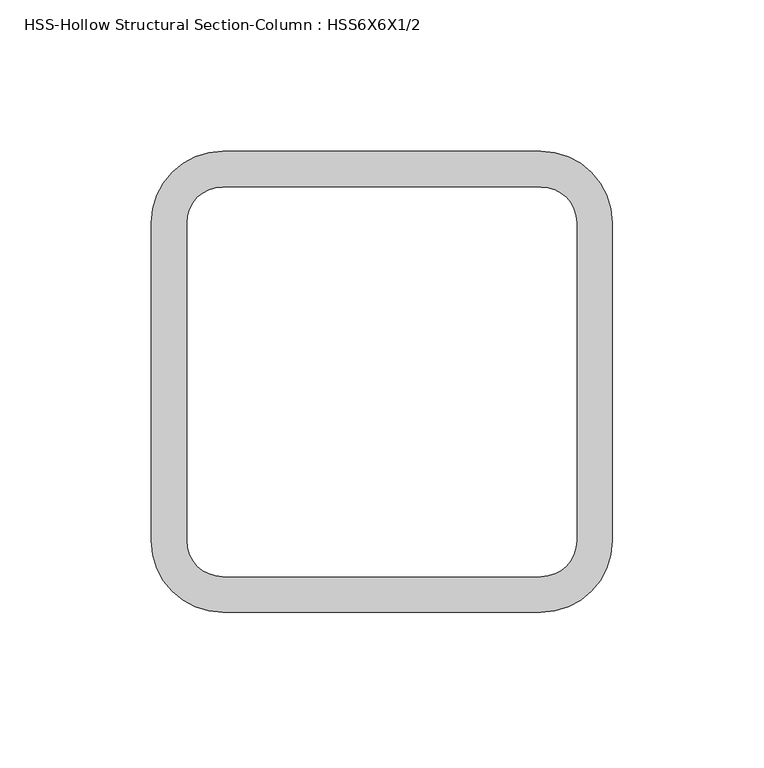
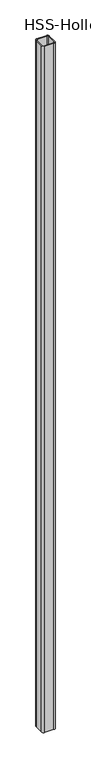
"""IFC4 building model written with IfcOpenShell, lengths in millimetres: column geometry, HSS-Hollow Structural Section-Column : HSS6X6X1/2."""

from ifc_helpers import new_model, si_unit, point, frame, frame_2d, origin, place, context, project, spatial, polyline, circle_curve, trimmed, segment, composite_curve, outline, extrude, source, transform, mapped, element, save


def hss_hollow_structural_section_column_hss6x6x1_2_eccfc461(model_context):
    return source(origin(), model_context, "Body", "SweptSolid", [
        extrude(outline(composite_curve([segment(trimmed(circle_curve(frame_2d((52.578, 52.578)), 23.622), [point((52.578, 76.2))], [point((76.2, 52.578))], False, "CARTESIAN"), True, "CONTINUOUS"), segment(polyline([(76.2, 52.578), (76.2, -52.578)]), True, "CONTINUOUS"), segment(trimmed(circle_curve(frame_2d((52.578, -52.578)), 23.622), [point((76.2, -52.578))], [point((52.578, -76.2))], False, "CARTESIAN"), True, "CONTINUOUS"), segment(polyline([(52.578, -76.2), (-52.578, -76.2)]), True, "CONTINUOUS"), segment(trimmed(circle_curve(frame_2d((-52.578, -52.578)), 23.622), [point((-52.578, -76.2))], [point((-76.2, -52.578))], False, "CARTESIAN"), True, "CONTINUOUS"), segment(polyline([(-76.2, -52.578), (-76.2, 52.578)]), True, "CONTINUOUS"), segment(trimmed(circle_curve(frame_2d((-52.578, 52.578)), 23.622), [point((-76.2, 52.578))], [point((-52.578, 76.2))], False, "CARTESIAN"), True, "CONTINUOUS"), segment(polyline([(-52.578, 76.2), (52.578, 76.2)]), True, "CONTINUOUS")], self_intersect=False), holes=[composite_curve([segment(polyline([(52.578, 64.389), (-52.578, 64.389)]), True, "CONTINUOUS"), segment(trimmed(circle_curve(frame_2d((-52.578, 52.578)), 11.811), [point((-52.578, 64.389))], [point((-64.389, 52.578))], True, "CARTESIAN"), True, "CONTINUOUS"), segment(polyline([(-64.389, 52.578), (-64.389, -52.578)]), True, "CONTINUOUS"), segment(trimmed(circle_curve(frame_2d((-52.578, -52.578)), 11.811), [point((-64.389, -52.578))], [point((-52.578, -64.389))], True, "CARTESIAN"), True, "CONTINUOUS"), segment(polyline([(-52.578, -64.389), (52.578, -64.389)]), True, "CONTINUOUS"), segment(trimmed(circle_curve(frame_2d((52.578, -52.578)), 11.811), [point((52.578, -64.389))], [point((64.389, -52.578))], True, "CARTESIAN"), True, "CONTINUOUS"), segment(polyline([(64.389, -52.578), (64.389, 52.578)]), True, "CONTINUOUS"), segment(trimmed(circle_curve(frame_2d((52.578, 52.578)), 11.811), [point((64.389, 52.578))], [point((52.578, 64.389))], True, "CARTESIAN"), True, "CONTINUOUS")], self_intersect=False)]), frame((0.0, 0.0, 4267.2), z_axis=(0.0, 0.0, 1.0), x_axis=(1.0, 0.0, 0.0)), (0.0, 0.0, 1.0), 8280.4),
    ])


if __name__ == "__main__":
    model = new_model("IFC4")
    model_context = context("Model", 3, world=origin())
    ifc_project = project(units=[si_unit("LENGTHUNIT", "METRE", prefix="MILLI")], contexts=[model_context])
    site = spatial("IfcSite", under=ifc_project)
    building = spatial("IfcBuilding", under=site)
    placement = place(None, origin())
    hss_hollow_structural_section_column_hss6x6x1_2_shape = hss_hollow_structural_section_column_hss6x6x1_2_eccfc461(model_context)
    element("IfcColumn", 1, ObjectType="HSS-Hollow Structural Section-Column : HSS6X6X1/2", at=placement, inside=building, context=model_context, shape_type="MappedRepresentation", body=[
        mapped(hss_hollow_structural_section_column_hss6x6x1_2_shape, transform((0.0, 0.0, 0.0), x_axis=(1.0, 0.0, 0.0), y_axis=(0.0, 1.0, 0.0), z_axis=(0.0, 0.0, 1.0))),
    ])
    save(model, "model.ifc")

# Revit data of these elements
# Type "HSS-Hollow Structural Section-Column : HSS6X6X1/2"
#   Assembly Code = "B10"
#   Shape = "Square"
#   W = 35.1
#   Ht = 0' - 6"
#   b = 0' - 6"
#   kr = 0' - 0.93"
#   t = 0' - 0.465"
#   A = 0.0676389 SF
#   Structural Material [instance default] = Steel ASTM A500, Grade B, Rectangular and Square
# Element 1 (IfcColumn, "HSS-Hollow Structural Section-Column : HSS6X6X1/2")
#   Materials on its faces: "Steel ASTM A500, Grade B, Rectangular and Square"
# Materials
#   "Steel ASTM A500, Grade B, Rectangular and Square": class "Metal", colour RGB 199 199 199, transparency 0, Description = "Carbon steel", Cost = 0
